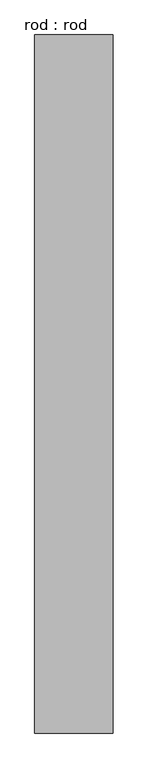
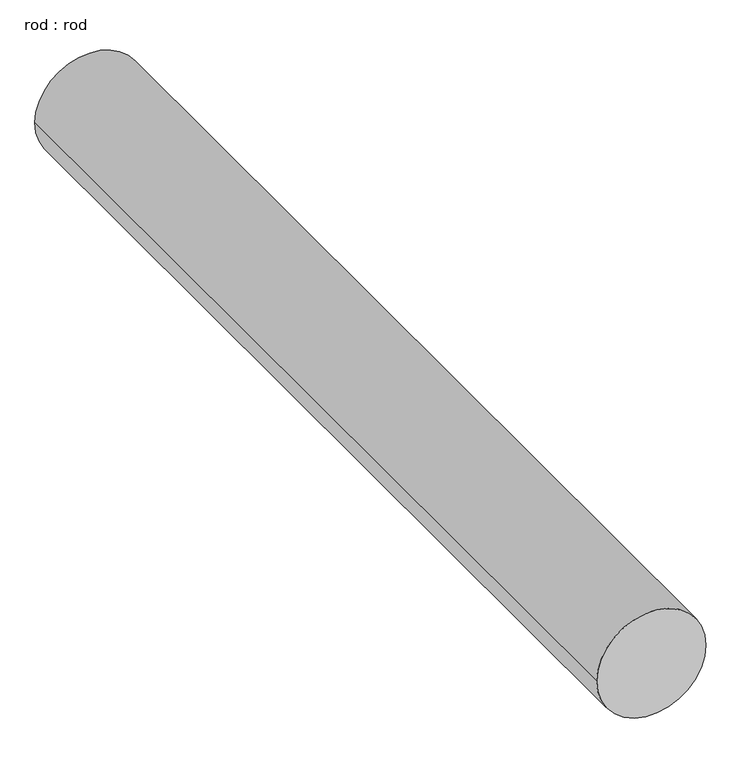
"""IFC4 building model written with IfcOpenShell, lengths in millimetres: proxy geometry, rod : rod."""

from ifc_helpers import new_model, si_unit, point, frame, frame_2d, origin, place, context, project, spatial, circle_curve, trimmed, segment, composite_curve, outline, extrude, source, transform, mapped, element, save


def rod_rod_a408fcd6(model_context):
    return source(origin(), model_context, "Body", "SweptSolid", [
        extrude(outline(composite_curve([segment(trimmed(circle_curve(frame_2d((0.0108462, 0.0)), 200.0), [point((0.0108462, 200.0))], [point((0.0108462, -200.0))], False, "CARTESIAN"), True, "CONTINUOUS"), segment(trimmed(circle_curve(frame_2d((0.0108462, 0.0)), 200.0), [point((0.0108462, -200.0))], [point((0.0108462, 200.0))], False, "CARTESIAN"), True, "CONTINUOUS")], self_intersect=False)), frame((0.0, 2312.7286153, 0.0), z_axis=(0.0, 1.0, 0.0), x_axis=(0.0, 0.0, 1.0)), (0.0, 0.0, 1.0), 3560.0),
    ])


if __name__ == "__main__":
    model = new_model("IFC4")
    model_context = context("Model", 3, world=origin())
    ifc_project = project(units=[si_unit("LENGTHUNIT", "METRE", prefix="MILLI")], contexts=[model_context])
    site = spatial("IfcSite", under=ifc_project)
    building = spatial("IfcBuilding", under=site)
    placement = place(None, origin())
    rod_rod_shape = rod_rod_a408fcd6(model_context)
    element("IfcBuildingElementProxy", 1, Name="rod : rod", ObjectType="rod : rod", at=placement, inside=building, context=model_context, shape_type="MappedRepresentation", body=[
        mapped(rod_rod_shape, transform((0.0, 0.0, 0.0), x_axis=(1.0, 0.0, 0.0), y_axis=(0.0, 1.0, 0.0), z_axis=(0.0, 0.0, 1.0))),
    ])
    save(model, "model.ifc")

# Revit data of these elements
# Type "rod : rod"
#   Default Elevation = 0
